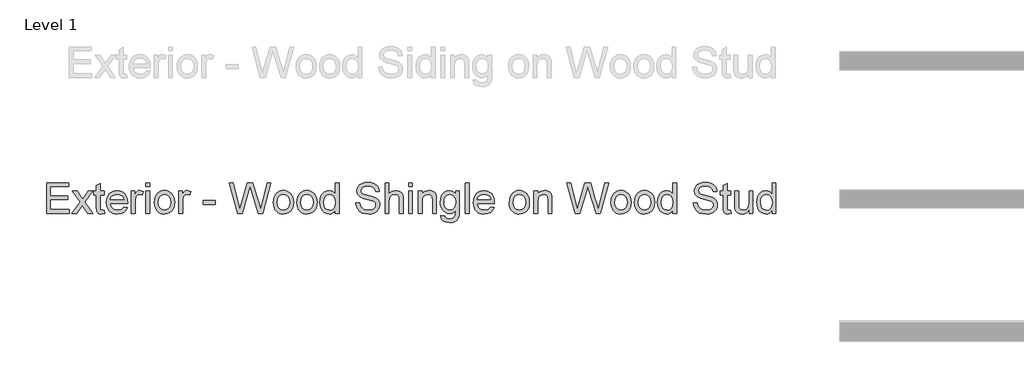
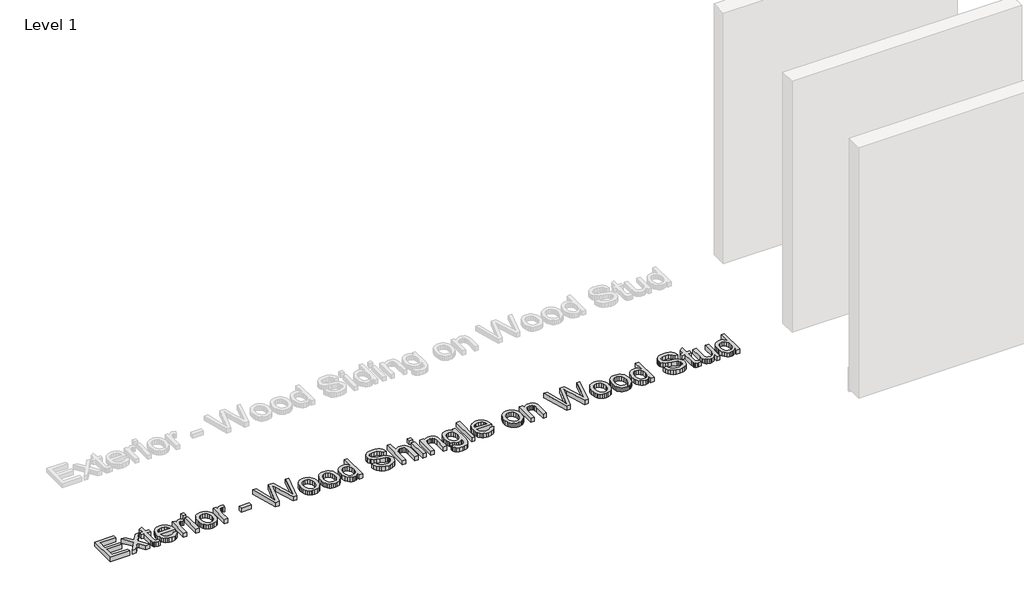
# One storey, part 30 of 42: 1 proxy.
"""IFC4 building model written with IfcOpenShell, lengths in millimetres."""

from ifc_helpers import new_model, si_unit, origin, origin_with_axes, place, context, project, spatial, polyline, outline, extrude, element, save

model = new_model("IFC4")

# Units and contexts
model_context = context("Model", 3, world=origin())
ifc_project = project(units=[si_unit("LENGTHUNIT", "METRE", prefix="MILLI")], contexts=[model_context])

# Site, building, storey
site = spatial("IfcSite", under=ifc_project)
building = spatial("IfcBuilding", under=site)
storey = spatial("IfcBuildingStorey", under=building, Name="Level 1", Elevation=0.0)

# Proxy
placement = place(None, origin())
element("IfcBuildingElementProxy", 1, Name="8\" Arial", ObjectType="8\" Arial", at=placement, inside=storey, context=model_context, shape_type="SweptSolid", body=[
    extrude(outline(polyline([(-7203.1148942, 15956.5861891), (-7203.1148942, 16261.1532832), (-6984.2072954, 16261.1532832), (-6984.2072954, 16223.0823964), (-7165.0440075, 16223.0823964), (-7165.0440075, 16132.6640404), (-6993.7250171, 16132.6640404), (-6993.7250171, 16094.5931536), (-7165.0440075, 16094.5931536), (-7165.0440075, 15994.6570759), (-6979.4484345, 15994.6570759), (-6979.4484345, 15956.5861891), (-7203.1148942, 15956.5861891)])), origin_with_axes(), (0.0, 0.0, 1.0), 50.8),
    extrude(outline(polyline([(-6950.8952695, 15956.5861891), (-6869.5484919, 16069.0142766), (-6946.1364086, 16180.2526488), (-6900.332373, 16180.2526488), (-6863.3768442, 16126.7154643), (-6846.1259737, 16101.4340161), (-6831.1801763, 16122.1053179), (-6789.0940008, 16180.2526488), (-6743.2899651, 16180.2526488), (-6823.7444563, 16069.0142766), (-6746.2642531, 15956.5861891), (-6792.0682888, 15956.5861891), (-6838.6902536, 16024.1768845), (-6847.2413317, 16036.5201799), (-6905.0912338, 15956.5861891), (-6950.8952695, 15956.5861891)])), origin_with_axes(), (0.0, 0.0, 1.0), 50.8),
    extrude(outline(polyline([(-6632.0515929, 15988.3367138), (-6627.292732, 15955.4708311), (-6655.7715399, 15951.8273283), (-6674.044822, 15953.4074188), (-6687.670779, 15958.1476903), (-6697.3000365, 15965.4532853), (-6703.5832199, 15974.7293461), (-6707.0408298, 15990.6603763), (-6708.1933664, 16017.9308797), (-6708.1933664, 16142.1817621), (-6736.7465315, 16142.1817621), (-6736.7465315, 16180.2526488), (-6708.1933664, 16180.2526488), (-6708.1933664, 16234.6077625), (-6670.1224796, 16256.9892799), (-6670.1224796, 16180.2526488), (-6632.0515929, 16180.2526488), (-6632.0515929, 16142.1817621), (-6670.1224796, 16142.1817621), (-6670.1224796, 16019.0462377), (-6668.1148352, 15999.4159367), (-6661.6085801, 15992.4635384), (-6648.6332486, 15989.898215), (-6632.0515929, 15988.3367138)])), origin_with_axes(), (0.0, 0.0, 1.0), 50.8),
    extrude(outline(polyline([(-6437.3844414, 16023.2102409), (-6400.0571267, 16018.4513801), (-6413.5064854, 15990.3257689), (-6434.9678324, 15969.3012704), (-6463.957846, 15956.1958138), (-6499.9932044, 15951.8273283), (-6523.6155576, 15953.7118186), (-6544.6632927, 15959.3652895), (-6563.1364098, 15968.787741), (-6579.0349088, 15981.9791732), (-6591.8197, 15998.5724472), (-6600.9516937, 16018.2004245), (-6606.4308899, 16040.8631051), (-6608.2572886, 16066.5604889), (-6606.4123006, 16093.1292462), (-6600.8773365, 16116.5471171), (-6591.6523963, 16136.8141016), (-6578.73748, 16153.9301998), (-6562.8808069, 16167.5282728), (-6544.8305964, 16177.2411822), (-6524.5868486, 16183.0689278), (-6502.1495632, 16185.0115097), (-6480.434937, 16183.0735751), (-6460.797665, 16177.2597715), (-6443.2377473, 16167.5700988), (-6427.7551839, 16154.004557), (-6415.1167835, 16136.9256374), (-6406.0893546, 16116.6958315), (-6400.6728973, 16093.3151392), (-6398.8674115, 16066.7835605), (-6399.0904831, 16056.5222669), (-6570.1864019, 16056.5222669), (-6563.596495, 16028.0248697), (-6548.2882063, 16007.0747284), (-6526.194823, 15994.1923434), (-6499.2496324, 15989.898215), (-6478.9872952, 15991.8872701), (-6461.9223177, 15997.8544355), (-6448.0546997, 16008.1714971), (-6437.3844414, 16023.2102409)]), holes=[polyline([(-6570.1864019, 16094.5931536), (-6436.9382982, 16094.5931536), (-6442.0875344, 16114.7067764), (-6452.1815244, 16129.0948947), (-6474.3771488, 16142.4791909), (-6502.2982776, 16146.9406229), (-6527.9608065, 16143.3807719), (-6549.1804927, 16132.701219), (-6563.9311024, 16116.0545007), (-6570.1864019, 16094.5931536)])]), origin_with_axes(), (0.0, 0.0, 1.0), 50.8),
    extrude(outline(polyline([(-6360.7965247, 15956.5861891), (-6360.7965247, 16180.2526488), (-6327.4844988, 16180.2526488), (-6327.4844988, 16147.1636945), (-6315.1783821, 16166.3478523), (-6303.838909, 16177.6501468), (-6292.4622573, 16183.1711689), (-6280.0446048, 16185.0115097), (-6261.0835186, 16182.0744002), (-6241.8250036, 16173.263072), (-6254.5400849, 16139.1331168), (-6267.924381, 16144.9887464), (-6281.3086772, 16146.9406229), (-6292.6760342, 16145.0631036), (-6302.8350868, 16139.4305456), (-6311.0422628, 16130.4705029), (-6316.5539903, 16118.6105294), (-6321.182726, 16097.34437), (-6322.725638, 16074.1449234), (-6322.725638, 15956.5861891), (-6360.7965247, 15956.5861891)])), origin_with_axes(), (0.0, 0.0, 1.0), 50.8),
    extrude(outline(polyline([(-6218.0306994, 16223.0823964), (-6218.0306994, 16261.1532832), (-6179.9598126, 16261.1532832), (-6179.9598126, 16223.0823964), (-6218.0306994, 16223.0823964)])), origin_with_axes(), (0.0, 0.0, 1.0), 50.8),
    extrude(outline(polyline([(-6218.0306994, 15956.5861891), (-6218.0306994, 16180.2526488), (-6179.9598126, 16180.2526488), (-6179.9598126, 15956.5861891), (-6218.0306994, 15956.5861891)])), origin_with_axes(), (0.0, 0.0, 1.0), 50.8),
    extrude(outline(polyline([(-6132.3712042, 16068.419419), (-6130.3124392, 16097.386196), (-6124.1361442, 16122.3469788), (-6113.8423192, 16143.3017674), (-6099.4309643, 16160.2505618), (-6084.9220155, 16171.0834765), (-6068.9073334, 16178.8212727), (-6051.386918, 16183.4639504), (-6032.3607692, 16185.0115097), (-6011.3571837, 16183.1270194), (-5992.3658899, 16177.4735484), (-5975.3868878, 16168.0510969), (-5960.4201775, 16154.8596648), (-5948.2046837, 16138.3453952), (-5939.4793309, 16118.9544315), (-5934.2441192, 16096.6867735), (-5932.4990487, 16071.5424214), (-5935.5848725, 16033.0811593), (-5944.842344, 16003.8030116), (-5960.0019183, 15981.876932), (-5980.7940505, 15965.4718746), (-6005.4899358, 15955.2384648), (-6032.3607692, 15951.8273283), (-6053.6710782, 15953.7048476), (-6072.8389704, 15959.3374055), (-6089.8644457, 15968.7250021), (-6104.7475041, 15981.8676373), (-6116.8328729, 15998.5422396), (-6125.4652792, 16018.5257373), (-6130.6447229, 16041.8181304), (-6132.3712042, 16068.419419)]), holes=[polyline([(-6094.3003174, 16068.4937762), (-6089.8946533, 16034.0385083), (-6076.6776608, 16009.4913374), (-6056.7871097, 15994.7964956), (-6032.3607692, 15989.898215), (-6008.0459646, 15994.8243796), (-5988.192592, 16009.6028732), (-5974.9755996, 16034.4753568), (-5970.5699354, 16069.6834914), (-5975.0034835, 16103.134937), (-5988.3041278, 16127.3475005), (-6008.1853843, 16142.0423423), (-6032.3607692, 16146.9406229), (-6056.7871097, 16142.0609316), (-6076.6776608, 16127.4218577), (-6089.8946533, 16102.9304547), (-6094.3003174, 16068.4937762)])]), origin_with_axes(), (0.0, 0.0, 1.0), 50.8),
    extrude(outline(polyline([(-5889.6693011, 15956.5861891), (-5889.6693011, 16180.2526488), (-5856.3572752, 16180.2526488), (-5856.3572752, 16147.1636945), (-5844.0511585, 16166.3478523), (-5832.7116853, 16177.6501468), (-5821.3350336, 16183.1711689), (-5808.9173811, 16185.0115097), (-5789.9562949, 16182.0744002), (-5770.69778, 16173.263072), (-5783.4128613, 16139.1331168), (-5796.7971574, 16144.9887464), (-5810.1814535, 16146.9406229), (-5821.5488106, 16145.0631036), (-5831.7078631, 16139.4305456), (-5839.9150392, 16130.4705029), (-5845.4267667, 16118.6105294), (-5850.0555024, 16097.34437), (-5851.5984143, 16074.1449234), (-5851.5984143, 15956.5861891), (-5889.6693011, 15956.5861891)])), origin_with_axes(), (0.0, 0.0, 1.0), 50.8),
    extrude(outline(polyline([(-5646.967398, 16047.0045452), (-5646.967398, 16085.0754319), (-5527.9958769, 16085.0754319), (-5527.9958769, 16047.0045452), (-5646.967398, 16047.0045452)])), origin_with_axes(), (0.0, 0.0, 1.0), 50.8),
    extrude(outline(polyline([(-5306.9319192, 15956.5861891), (-5389.9889124, 16261.1532832), (-5350.7283104, 16261.1532832), (-5302.5448444, 16060.9836989), (-5287.6734042, 15999.1928651), (-5271.7609633, 16053.8454076), (-5211.3829163, 16261.1532832), (-5154.7970866, 16261.1532832), (-5110.9263381, 16110.8773806), (-5092.1325557, 16055.10948), (-5078.283527, 15999.1928651), (-5063.8582301, 16059.1991261), (-5015.2286208, 16261.1532832), (-4975.9680189, 16261.1532832), (-5059.0993693, 15956.5861891), (-5099.772758, 15956.5861891), (-5172.7915291, 16191.5549433), (-5182.9784656, 16224.3464688), (-5194.4294745, 16184.8627953), (-5260.9791692, 15956.5861891), (-5306.9319192, 15956.5861891)])), origin_with_axes(), (0.0, 0.0, 1.0), 50.8),
    extrude(outline(polyline([(-4952.1737147, 16068.419419), (-4950.1149497, 16097.386196), (-4943.9386547, 16122.3469788), (-4933.6448297, 16143.3017674), (-4919.2334747, 16160.2505618), (-4904.724526, 16171.0834765), (-4888.7098439, 16178.8212727), (-4871.1894284, 16183.4639504), (-4852.1632797, 16185.0115097), (-4831.1596942, 16183.1270194), (-4812.1684004, 16177.4735484), (-4795.1893983, 16168.0510969), (-4780.222688, 16154.8596648), (-4768.0071942, 16138.3453952), (-4759.2818414, 16118.9544315), (-4754.0466297, 16096.6867735), (-4752.3015592, 16071.5424214), (-4755.387383, 16033.0811593), (-4764.6448545, 16003.8030116), (-4779.8044288, 15981.876932), (-4800.596561, 15965.4718746), (-4825.2924463, 15955.2384648), (-4852.1632797, 15951.8273283), (-4873.4735887, 15953.7048476), (-4892.6414808, 15959.3374055), (-4909.6669561, 15968.7250021), (-4924.5500146, 15981.8676373), (-4936.6353834, 15998.5422396), (-4945.2677896, 16018.5257373), (-4950.4472334, 16041.8181304), (-4952.1737147, 16068.419419)]), holes=[polyline([(-4914.1028279, 16068.4937762), (-4909.6971638, 16034.0385083), (-4896.4801713, 16009.4913374), (-4876.5896201, 15994.7964956), (-4852.1632797, 15989.898215), (-4827.8484751, 15994.8243796), (-4807.9951025, 16009.6028732), (-4794.7781101, 16034.4753568), (-4790.3724459, 16069.6834914), (-4794.805994, 16103.134937), (-4808.1066383, 16127.3475005), (-4827.9878948, 16142.0423423), (-4852.1632797, 16146.9406229), (-4876.5896201, 16142.0609316), (-4896.4801713, 16127.4218577), (-4909.6971638, 16102.9304547), (-4914.1028279, 16068.4937762)])]), origin_with_axes(), (0.0, 0.0, 1.0), 50.8),
    extrude(outline(polyline([(-4718.9895333, 16068.419419), (-4716.9307683, 16097.386196), (-4710.7544733, 16122.3469788), (-4700.4606483, 16143.3017674), (-4686.0492933, 16160.2505618), (-4671.5403446, 16171.0834765), (-4655.5256625, 16178.8212727), (-4638.005247, 16183.4639504), (-4618.9790983, 16185.0115097), (-4597.9755128, 16183.1270194), (-4578.984219, 16177.4735484), (-4562.0052169, 16168.0510969), (-4547.0385066, 16154.8596648), (-4534.8230128, 16138.3453952), (-4526.09766, 16118.9544315), (-4520.8624483, 16096.6867735), (-4519.1173778, 16071.5424214), (-4522.2032016, 16033.0811593), (-4531.4606731, 16003.8030116), (-4546.6202474, 15981.876932), (-4567.4123796, 15965.4718746), (-4592.1082649, 15955.2384648), (-4618.9790983, 15951.8273283), (-4640.2894073, 15953.7048476), (-4659.4572994, 15959.3374055), (-4676.4827747, 15968.7250021), (-4691.3658332, 15981.8676373), (-4703.451202, 15998.5422396), (-4712.0836082, 16018.5257373), (-4717.263052, 16041.8181304), (-4718.9895333, 16068.419419)]), holes=[polyline([(-4680.9186465, 16068.4937762), (-4676.5129824, 16034.0385083), (-4663.2959899, 16009.4913374), (-4643.4054387, 15994.7964956), (-4618.9790983, 15989.898215), (-4594.6642937, 15994.8243796), (-4574.8109211, 16009.6028732), (-4561.5939287, 16034.4753568), (-4557.1882645, 16069.6834914), (-4561.6218126, 16103.134937), (-4574.9224569, 16127.3475005), (-4594.8037134, 16142.0423423), (-4618.9790983, 16146.9406229), (-4643.4054387, 16142.0609316), (-4663.2959899, 16127.4218577), (-4676.5129824, 16102.9304547), (-4680.9186465, 16068.4937762)])]), origin_with_axes(), (0.0, 0.0, 1.0), 50.8),
    extrude(outline(polyline([(-4338.2806657, 15956.5861891), (-4338.2806657, 15992.5007171), (-4349.6712594, 15974.7061095), (-4363.4691674, 15961.9956755), (-4379.6743898, 15954.3694151), (-4398.2869266, 15951.8273283), (-4422.8991601, 15955.5080097), (-4445.4293919, 15966.550054), (-4464.5020139, 15984.1820052), (-4478.7414178, 16007.6324074), (-4487.608514, 16035.9532062), (-4490.5642127, 16068.1963474), (-4487.8408802, 16100.0398186), (-4479.6708828, 16128.7974659), (-4466.0635151, 16152.8334311), (-4447.0280717, 16170.5118555), (-4424.0052234, 16181.3865961), (-4398.435641, 16185.0115097), (-4379.8091623, 16182.4183023), (-4363.3390423, 16174.6386802), (-4349.3784779, 16162.7136441), (-4338.2806657, 16147.6841949), (-4338.2806657, 16261.1532832), (-4300.2097789, 16261.1532832), (-4300.2097789, 15956.5861891), (-4338.2806657, 15956.5861891)]), holes=[polyline([(-4452.4933259, 16068.3450618), (-4448.1991976, 16033.9083832), (-4435.3168126, 16009.4169802), (-4416.5973873, 15994.7779063), (-4394.7921382, 15989.898215), (-4372.9961837, 15994.5548347), (-4354.7507856, 16008.5246938), (-4342.3981957, 16032.0680425), (-4338.2806657, 16065.4451309), (-4342.4725529, 16101.9359272), (-4355.0482144, 16127.2359647), (-4373.7583451, 16142.0144584), (-4396.3536394, 16146.9406229), (-4418.3819601, 16142.209646), (-4436.4321706, 16128.0167153), (-4448.4780371, 16103.6368481), (-4452.4933259, 16068.3450618)])]), origin_with_axes(), (0.0, 0.0, 1.0), 50.8),
    extrude(outline(polyline([(-4133.6496493, 16061.2811277), (-4095.5787626, 16061.2811277), (-4091.210277, 16040.154388), (-4083.3098245, 16023.1730623), (-4070.9851185, 16009.6958197), (-4053.3438726, 15999.0813293), (-4031.7802844, 15992.1939936), (-4007.6885514, 15989.898215), (-3986.4781599, 15991.6363146), (-3967.907449, 15996.8506133), (-3952.8594105, 16005.1042626), (-3942.2170361, 16015.9604139), (-3935.8873794, 16028.4245396), (-3933.7774939, 16041.5021123), (-3935.3575844, 16054.2450776), (-3940.0978559, 16065.2592379), (-3949.7271134, 16074.6561292), (-3965.9741618, 16082.5472871), (-4021.4074549, 16097.0841198), (-4057.79601, 16106.7040827), (-4081.0791084, 16115.859313), (-4100.0309, 16128.6673408), (-4113.4616694, 16144.1894065), (-4121.4643631, 16162.0909025), (-4124.1319277, 16182.0372216), (-4120.8323269, 16204.3350872), (-4110.9335245, 16225.1272194), (-4094.6957708, 16242.749876), (-4072.379316, 16255.5393145), (-4045.5921344, 16263.3189367), (-4015.9422006, 16265.912144), (-3983.8198899, 16263.1981062), (-3955.7128681, 16255.0559927), (-3932.6249572, 16241.6531073), (-3915.5599797, 16223.1567536), (-3904.7595963, 16200.7194683), (-3900.4654679, 16175.493788), (-3938.5363547, 16175.493788), (-3945.5259316, 16198.2099128), (-3960.0999429, 16214.6056755), (-3982.8718356, 16224.5323618), (-4014.4550566, 16227.8412573), (-4046.7818496, 16224.5695404), (-4068.9588847, 16214.7543899), (-4081.7855019, 16200.3105037), (-4086.0610409, 16183.1525796), (-4083.030985, 16168.5228004), (-4073.9408172, 16156.7557734), (-4052.4515862, 16146.2342295), (-4011.7781974, 16135.489614), (-3969.8035576, 16125.2840882), (-3944.4105736, 16116.3798134), (-3922.7075656, 16102.5679634), (-3907.5665806, 16085.5215751), (-3898.6716005, 16065.4265416), (-3895.7066071, 16042.4687559), (-3899.1177437, 16018.9997644), (-3909.3511534, 15996.9249705), (-3925.9885771, 15977.9267057), (-3948.6117554, 15963.6873018), (-3975.8171962, 15954.7923216), (-4006.2014073, 15951.8273283), (-4043.5008381, 15955.0246879), (-4074.2010674, 15964.6167668), (-4098.6552918, 15980.6407435), (-4117.216708, 16003.1337968), (-4129.1324494, 16030.5344252), (-4133.6496493, 16061.2811277)])), origin_with_axes(), (0.0, 0.0, 1.0), 50.8),
    extrude(outline(polyline([(-3843.3591378, 15956.5861891), (-3843.3591378, 16261.1532832), (-3805.288251, 16261.1532832), (-3805.288251, 16149.1713389), (-3791.30445, 16164.8514136), (-3775.6011387, 16176.051467), (-3758.1783171, 16182.771499), (-3739.0359852, 16185.0115097), (-3716.0410209, 16182.5670167), (-3696.2805948, 16175.2335378), (-3680.7213506, 16163.5873412), (-3670.3299318, 16148.2046953), (-3664.4743022, 16127.068661), (-3662.5224257, 16098.1622992), (-3662.5224257, 15956.5861891), (-3700.5933125, 15956.5861891), (-3700.5933125, 16094.2213676), (-3703.6233684, 16118.0528504), (-3712.7135362, 16134.374256), (-3727.3619047, 16143.7990312), (-3747.0665629, 16146.9406229), (-3763.1556022, 16144.8214427), (-3778.2594086, 16138.463902), (-3790.7700076, 16128.4814478), (-3799.0794248, 16115.487527), (-3803.7360445, 16098.2180671), (-3805.288251, 16075.4089958), (-3805.288251, 15956.5861891), (-3843.3591378, 15956.5861891)])), origin_with_axes(), (0.0, 0.0, 1.0), 50.8),
    extrude(outline(polyline([(-3610.1749564, 16223.0823964), (-3610.1749564, 16261.1532832), (-3572.1040697, 16261.1532832), (-3572.1040697, 16223.0823964), (-3610.1749564, 16223.0823964)])), origin_with_axes(), (0.0, 0.0, 1.0), 50.8),
    extrude(outline(polyline([(-3610.1749564, 15956.5861891), (-3610.1749564, 16180.2526488), (-3572.1040697, 16180.2526488), (-3572.1040697, 15956.5861891), (-3610.1749564, 15956.5861891)])), origin_with_axes(), (0.0, 0.0, 1.0), 50.8),
    extrude(outline(polyline([(-3514.9977395, 15956.5861891), (-3514.9977395, 16180.2526488), (-3476.9268528, 16180.2526488), (-3476.9268528, 16149.0226245), (-3463.7005657, 16164.7677618), (-3447.8160087, 16176.0142884), (-3429.2731818, 16182.7622043), (-3408.0720849, 16185.0115097), (-3389.3061864, 16183.1990529), (-3372.1203784, 16177.7616826), (-3357.7880279, 16169.3779082), (-3347.5825021, 16158.7262392), (-3336.1686718, 16130.7307532), (-3334.1610274, 16093.9239388), (-3334.1610274, 15956.5861891), (-3372.2319142, 15956.5861891), (-3372.2319142, 16088.793292), (-3376.618989, 16122.4771039), (-3382.6883955, 16132.5060313), (-3392.1224654, 16140.2856534), (-3404.2148051, 16145.2768805), (-3418.2590214, 16146.9406229), (-3440.556887, 16143.2041736), (-3459.5644464, 16131.9948256), (-3467.1604992, 16122.8442426), (-3472.5862512, 16110.3382909), (-3476.9268528, 16075.2602814), (-3476.9268528, 15956.5861891), (-3514.9977395, 15956.5861891)])), origin_with_axes(), (0.0, 0.0, 1.0), 50.8),
    extrude(outline(polyline([(-3291.3312798, 15937.5507457), (-3253.2603931, 15932.7918849), (-3249.0592112, 15920.8947328), (-3240.9170977, 15912.7154407), (-3224.9117103, 15906.3579), (-3203.961569, 15904.2387198), (-3181.6172302, 15906.6367395), (-3164.9983958, 15913.8307987), (-3153.4730297, 15925.3561648), (-3146.4090956, 15940.7481054), (-3143.8065936, 15985.1393542), (-3156.4752017, 15972.6473445), (-3170.6123645, 15963.7244804), (-3186.218082, 15958.3707619), (-3203.2923542, 15956.5861891), (-3224.1658146, 15958.6635434), (-3242.5436615, 15964.8956063), (-3258.4258948, 15975.2823778), (-3271.8125146, 15989.8238578), (-3282.433976, 16007.269916), (-3290.0207341, 16026.370422), (-3294.572789, 16047.1253756), (-3296.0901407, 16069.534777), (-3293.3668082, 16100.2721848), (-3285.1968108, 16128.5372157), (-3271.8682825, 16152.489529), (-3253.6693577, 16170.2887839), (-3231.2227777, 16181.3308282), (-3205.1512842, 16185.0115097), (-3187.347382, 16182.929508), (-3171.1886328, 16176.6835032), (-3156.6750367, 16166.2734951), (-3143.8065936, 16151.6994837), (-3143.8065936, 16180.2526488), (-3105.7357069, 16180.2526488), (-3105.7357069, 15987.1469986), (-3108.3382089, 15942.5605621), (-3116.145715, 15913.1987625), (-3129.5950736, 15893.7264706), (-3149.1231335, 15878.8085572), (-3174.3023406, 15869.3280141), (-3204.705141, 15866.1678331), (-3240.1270525, 15870.6199705), (-3268.0202974, 15883.9763826), (-3278.5255757, 15894.0029864), (-3285.9124988, 15906.2742482), (-3290.1810669, 15920.790168), (-3291.3312798, 15937.5507457)]), holes=[polyline([(-3258.0192539, 16072.137279), (-3253.9574918, 16037.2172786), (-3241.7722055, 16013.2091974), (-3223.4524502, 15999.2951063), (-3200.987281, 15994.6570759), (-3178.6894154, 15999.2672223), (-3160.2767136, 16013.0976616), (-3147.9241236, 16036.7990194), (-3143.8065936, 16071.021921), (-3148.0449541, 16104.0272235), (-3160.7600354, 16127.7936437), (-3179.4422821, 16142.1538781), (-3201.5821386, 16146.9406229), (-3223.3223251, 16142.2282353), (-3241.5491339, 16128.0910725), (-3253.9017239, 16104.677849), (-3258.0192539, 16072.137279)])]), origin_with_axes(), (0.0, 0.0, 1.0), 50.8),
    extrude(outline(polyline([(-3048.6293767, 15956.5861891), (-3048.6293767, 16261.1532832), (-3010.55849, 16261.1532832), (-3010.55849, 15956.5861891), (-3048.6293767, 15956.5861891)])), origin_with_axes(), (0.0, 0.0, 1.0), 50.8),
    extrude(outline(polyline([(-2796.8558952, 16023.2102409), (-2759.5285804, 16018.4513801), (-2772.9779391, 15990.3257689), (-2794.4392861, 15969.3012704), (-2823.4292998, 15956.1958138), (-2859.4646581, 15951.8273283), (-2883.0870113, 15953.7118186), (-2904.1347465, 15959.3652895), (-2922.6078635, 15968.787741), (-2938.5063625, 15981.9791732), (-2951.2911537, 15998.5724472), (-2960.4231474, 16018.2004245), (-2965.9023436, 16040.8631051), (-2967.7287424, 16066.5604889), (-2965.8837543, 16093.1292462), (-2960.3487902, 16116.5471171), (-2951.12385, 16136.8141016), (-2938.2089337, 16153.9301998), (-2922.3522606, 16167.5282728), (-2904.3020502, 16177.2411822), (-2884.0583023, 16183.0689278), (-2861.621017, 16185.0115097), (-2839.9063907, 16183.0735751), (-2820.2691187, 16177.2597715), (-2802.709201, 16167.5700988), (-2787.2266377, 16154.004557), (-2774.5882372, 16136.9256374), (-2765.5608083, 16116.6958315), (-2760.144351, 16093.3151392), (-2758.3388652, 16066.7835605), (-2758.5619368, 16056.5222669), (-2929.6578556, 16056.5222669), (-2923.0679487, 16028.0248697), (-2907.75966, 16007.0747284), (-2885.6662767, 15994.1923434), (-2858.7210861, 15989.898215), (-2838.4587489, 15991.8872701), (-2821.3937714, 15997.8544355), (-2807.5261535, 16008.1714971), (-2796.8558952, 16023.2102409)]), holes=[polyline([(-2929.6578556, 16094.5931536), (-2796.4097519, 16094.5931536), (-2801.5589881, 16114.7067764), (-2811.6529781, 16129.0948947), (-2833.8486025, 16142.4791909), (-2861.7697314, 16146.9406229), (-2887.4322603, 16143.3807719), (-2908.6519464, 16132.701219), (-2923.4025561, 16116.0545007), (-2929.6578556, 16094.5931536)])]), origin_with_axes(), (0.0, 0.0, 1.0), 50.8),
    extrude(outline(polyline([(-2610.814179, 16068.419419), (-2608.755414, 16097.386196), (-2602.579119, 16122.3469788), (-2592.2852941, 16143.3017674), (-2577.8739391, 16160.2505618), (-2563.3649903, 16171.0834765), (-2547.3503082, 16178.8212727), (-2529.8298928, 16183.4639504), (-2510.8037441, 16185.0115097), (-2489.8001585, 16183.1270194), (-2470.8088647, 16177.4735484), (-2453.8298627, 16168.0510969), (-2438.8631524, 16154.8596648), (-2426.6476585, 16138.3453952), (-2417.9223057, 16118.9544315), (-2412.6870941, 16096.6867735), (-2410.9420235, 16071.5424214), (-2414.0278473, 16033.0811593), (-2423.2853188, 16003.8030116), (-2438.4448931, 15981.876932), (-2459.2370254, 15965.4718746), (-2483.9329107, 15955.2384648), (-2510.8037441, 15951.8273283), (-2532.114053, 15953.7048476), (-2551.2819452, 15959.3374055), (-2568.3074205, 15968.7250021), (-2583.1904789, 15981.8676373), (-2595.2758477, 15998.5422396), (-2603.908254, 16018.5257373), (-2609.0876977, 16041.8181304), (-2610.814179, 16068.419419)]), holes=[polyline([(-2572.7432922, 16068.4937762), (-2568.3376281, 16034.0385083), (-2555.1206357, 16009.4913374), (-2535.2300845, 15994.7964956), (-2510.8037441, 15989.898215), (-2486.4889394, 15994.8243796), (-2466.6355668, 16009.6028732), (-2453.4185744, 16034.4753568), (-2449.0129103, 16069.6834914), (-2453.4464584, 16103.134937), (-2466.7471026, 16127.3475005), (-2486.6283592, 16142.0423423), (-2510.8037441, 16146.9406229), (-2535.2300845, 16142.0609316), (-2555.1206357, 16127.4218577), (-2568.3376281, 16102.9304547), (-2572.7432922, 16068.4937762)])]), origin_with_axes(), (0.0, 0.0, 1.0), 50.8),
    extrude(outline(polyline([(-2368.1122759, 15956.5861891), (-2368.1122759, 16180.2526488), (-2330.0413892, 16180.2526488), (-2330.0413892, 16149.0226245), (-2316.8151021, 16164.7677618), (-2300.9305451, 16176.0142884), (-2282.3877182, 16182.7622043), (-2261.1866213, 16185.0115097), (-2242.4207228, 16183.1990529), (-2225.2349148, 16177.7616826), (-2210.9025643, 16169.3779082), (-2200.6970385, 16158.7262392), (-2189.2832082, 16130.7307532), (-2187.2755638, 16093.9239388), (-2187.2755638, 15956.5861891), (-2225.3464506, 15956.5861891), (-2225.3464506, 16088.793292), (-2229.7335254, 16122.4771039), (-2235.8029319, 16132.5060313), (-2245.2370018, 16140.2856534), (-2257.3293415, 16145.2768805), (-2271.3735578, 16146.9406229), (-2293.6714234, 16143.2041736), (-2312.6789828, 16131.9948256), (-2320.2750356, 16122.8442426), (-2325.7007876, 16110.3382909), (-2330.0413892, 16075.2602814), (-2330.0413892, 15956.5861891), (-2368.1122759, 15956.5861891)])), origin_with_axes(), (0.0, 0.0, 1.0), 50.8),
    extrude(outline(polyline([(-1956.6938844, 15956.5861891), (-2039.7508776, 16261.1532832), (-2000.4902757, 16261.1532832), (-1952.3068096, 16060.9836989), (-1937.4353695, 15999.1928651), (-1921.5229285, 16053.8454076), (-1861.1448815, 16261.1532832), (-1804.5590518, 16261.1532832), (-1760.6883034, 16110.8773806), (-1741.8945209, 16055.10948), (-1728.0454923, 15999.1928651), (-1713.6201954, 16059.1991261), (-1664.9905861, 16261.1532832), (-1625.7299841, 16261.1532832), (-1708.8613345, 15956.5861891), (-1749.5347233, 15956.5861891), (-1822.5534944, 16191.5549433), (-1832.7404309, 16224.3464688), (-1844.1914398, 16184.8627953), (-1910.7411344, 15956.5861891), (-1956.6938844, 15956.5861891)])), origin_with_axes(), (0.0, 0.0, 1.0), 50.8),
    extrude(outline(polyline([(-1601.9356799, 16068.419419), (-1599.8769149, 16097.386196), (-1593.7006199, 16122.3469788), (-1583.4067949, 16143.3017674), (-1568.99544, 16160.2505618), (-1554.4864912, 16171.0834765), (-1538.4718091, 16178.8212727), (-1520.9513937, 16183.4639504), (-1501.925245, 16185.0115097), (-1480.9216594, 16183.1270194), (-1461.9303656, 16177.4735484), (-1444.9513636, 16168.0510969), (-1429.9846533, 16154.8596648), (-1417.7691594, 16138.3453952), (-1409.0438066, 16118.9544315), (-1403.808595, 16096.6867735), (-1402.0635244, 16071.5424214), (-1405.1493482, 16033.0811593), (-1414.4068197, 16003.8030116), (-1429.566394, 15981.876932), (-1450.3585263, 15965.4718746), (-1475.0544116, 15955.2384648), (-1501.925245, 15951.8273283), (-1523.2355539, 15953.7048476), (-1542.4034461, 15959.3374055), (-1559.4289214, 15968.7250021), (-1574.3119798, 15981.8676373), (-1586.3973486, 15998.5422396), (-1595.0297549, 16018.5257373), (-1600.2091986, 16041.8181304), (-1601.9356799, 16068.419419)]), holes=[polyline([(-1563.8647931, 16068.4937762), (-1559.459129, 16034.0385083), (-1546.2421366, 16009.4913374), (-1526.3515854, 15994.7964956), (-1501.925245, 15989.898215), (-1477.6104403, 15994.8243796), (-1457.7570677, 16009.6028732), (-1444.5400753, 16034.4753568), (-1440.1344112, 16069.6834914), (-1444.5679593, 16103.134937), (-1457.8686035, 16127.3475005), (-1477.7498601, 16142.0423423), (-1501.925245, 16146.9406229), (-1526.3515854, 16142.0609316), (-1546.2421366, 16127.4218577), (-1559.459129, 16102.9304547), (-1563.8647931, 16068.4937762)])]), origin_with_axes(), (0.0, 0.0, 1.0), 50.8),
    extrude(outline(polyline([(-1368.7514985, 16068.419419), (-1366.6927335, 16097.386196), (-1360.5164385, 16122.3469788), (-1350.2226136, 16143.3017674), (-1335.8112586, 16160.2505618), (-1321.3023098, 16171.0834765), (-1305.2876277, 16178.8212727), (-1287.7672123, 16183.4639504), (-1268.7410636, 16185.0115097), (-1247.737478, 16183.1270194), (-1228.7461842, 16177.4735484), (-1211.7671822, 16168.0510969), (-1196.8004719, 16154.8596648), (-1184.584978, 16138.3453952), (-1175.8596252, 16118.9544315), (-1170.6244136, 16096.6867735), (-1168.879343, 16071.5424214), (-1171.9651668, 16033.0811593), (-1181.2226383, 16003.8030116), (-1196.3822126, 15981.876932), (-1217.1743449, 15965.4718746), (-1241.8702302, 15955.2384648), (-1268.7410636, 15951.8273283), (-1290.0513725, 15953.7048476), (-1309.2192647, 15959.3374055), (-1326.24474, 15968.7250021), (-1341.1277984, 15981.8676373), (-1353.2131672, 15998.5422396), (-1361.8455735, 16018.5257373), (-1367.0250172, 16041.8181304), (-1368.7514985, 16068.419419)]), holes=[polyline([(-1330.6806117, 16068.4937762), (-1326.2749476, 16034.0385083), (-1313.0579552, 16009.4913374), (-1293.167404, 15994.7964956), (-1268.7410636, 15989.898215), (-1244.4262589, 15994.8243796), (-1224.5728863, 16009.6028732), (-1211.3558939, 16034.4753568), (-1206.9502298, 16069.6834914), (-1211.3837779, 16103.134937), (-1224.6844221, 16127.3475005), (-1244.5656787, 16142.0423423), (-1268.7410636, 16146.9406229), (-1293.167404, 16142.0609316), (-1313.0579552, 16127.4218577), (-1326.2749476, 16102.9304547), (-1330.6806117, 16068.4937762)])]), origin_with_axes(), (0.0, 0.0, 1.0), 50.8),
    extrude(outline(polyline([(-988.0426309, 15956.5861891), (-988.0426309, 15992.5007171), (-999.4332246, 15974.7061095), (-1013.2311327, 15961.9956755), (-1029.4363551, 15954.3694151), (-1048.0488919, 15951.8273283), (-1072.6611253, 15955.5080097), (-1095.1913571, 15966.550054), (-1114.2639791, 15984.1820052), (-1128.503383, 16007.6324074), (-1137.3704792, 16035.9532062), (-1140.326178, 16068.1963474), (-1137.6028455, 16100.0398186), (-1129.432848, 16128.7974659), (-1115.8254803, 16152.8334311), (-1096.7900369, 16170.5118555), (-1073.7671887, 16181.3865961), (-1048.1976063, 16185.0115097), (-1029.5711275, 16182.4183023), (-1013.1010076, 16174.6386802), (-999.1404431, 16162.7136441), (-988.0426309, 16147.6841949), (-988.0426309, 16261.1532832), (-949.9717442, 16261.1532832), (-949.9717442, 15956.5861891), (-988.0426309, 15956.5861891)]), holes=[polyline([(-1102.2552912, 16068.3450618), (-1097.9611629, 16033.9083832), (-1085.0787778, 16009.4169802), (-1066.3593526, 15994.7779063), (-1044.5541035, 15989.898215), (-1022.758149, 15994.5548347), (-1004.5127509, 16008.5246938), (-992.1601609, 16032.0680425), (-988.0426309, 16065.4451309), (-992.2345181, 16101.9359272), (-1004.8101797, 16127.2359647), (-1023.5203103, 16142.0144584), (-1046.1156047, 16146.9406229), (-1068.1439254, 16142.209646), (-1086.1941358, 16128.0167153), (-1098.2400024, 16103.6368481), (-1102.2552912, 16068.3450618)])]), origin_with_axes(), (0.0, 0.0, 1.0), 50.8),
    extrude(outline(polyline([(-783.4116146, 16061.2811277), (-745.3407278, 16061.2811277), (-740.9722423, 16040.154388), (-733.0717897, 16023.1730623), (-720.7470837, 16009.6958197), (-703.1058378, 15999.0813293), (-681.5422496, 15992.1939936), (-657.4505166, 15989.898215), (-636.2401251, 15991.6363146), (-617.6694142, 15996.8506133), (-602.6213757, 16005.1042626), (-591.9790014, 16015.9604139), (-585.6493447, 16028.4245396), (-583.5394591, 16041.5021123), (-585.1195496, 16054.2450776), (-589.8598212, 16065.2592379), (-599.4890787, 16074.6561292), (-615.736127, 16082.5472871), (-671.1694201, 16097.0841198), (-707.5579752, 16106.7040827), (-730.8410737, 16115.859313), (-749.7928652, 16128.6673408), (-763.2236346, 16144.1894065), (-771.2263283, 16162.0909025), (-773.8938929, 16182.0372216), (-770.5942921, 16204.3350872), (-760.6954898, 16225.1272194), (-744.4577361, 16242.749876), (-722.1412812, 16255.5393145), (-695.3540997, 16263.3189367), (-665.7041659, 16265.912144), (-633.5818552, 16263.1981062), (-605.4748333, 16255.0559927), (-582.3869225, 16241.6531073), (-565.3219449, 16223.1567536), (-554.5215615, 16200.7194683), (-550.2274332, 16175.493788), (-588.29832, 16175.493788), (-595.2878968, 16198.2099128), (-609.8619082, 16214.6056755), (-632.6338009, 16224.5323618), (-664.2170219, 16227.8412573), (-696.5438149, 16224.5695404), (-718.72085, 16214.7543899), (-731.5474671, 16200.3105037), (-735.8230061, 16183.1525796), (-732.7929502, 16168.5228004), (-723.7027824, 16156.7557734), (-702.2135514, 16146.2342295), (-661.5401626, 16135.489614), (-619.5655228, 16125.2840882), (-594.1725388, 16116.3798134), (-572.4695309, 16102.5679634), (-557.3285459, 16085.5215751), (-548.4335657, 16065.4265416), (-545.4685723, 16042.4687559), (-548.8797089, 16018.9997644), (-559.1131187, 15996.9249705), (-575.7505423, 15977.9267057), (-598.3737206, 15963.6873018), (-625.5791615, 15954.7923216), (-655.9633726, 15951.8273283), (-693.2628034, 15955.0246879), (-723.9630326, 15964.6167668), (-748.417257, 15980.6407435), (-766.9786732, 16003.1337968), (-778.8944146, 16030.5344252), (-783.4116146, 16061.2811277)])), origin_with_axes(), (0.0, 0.0, 1.0), 50.8),
    extrude(outline(polyline([(-412.2204687, 15988.3367138), (-407.4616079, 15955.4708311), (-435.9404157, 15951.8273283), (-454.2136978, 15953.4074188), (-467.8396548, 15958.1476903), (-477.4689123, 15965.4532853), (-483.7520958, 15974.7293461), (-487.2097056, 15990.6603763), (-488.3622422, 16017.9308797), (-488.3622422, 16142.1817621), (-516.9154073, 16142.1817621), (-516.9154073, 16180.2526488), (-488.3622422, 16180.2526488), (-488.3622422, 16234.6077625), (-450.2913555, 16256.9892799), (-450.2913555, 16180.2526488), (-412.2204687, 16180.2526488), (-412.2204687, 16142.1817621), (-450.2913555, 16142.1817621), (-450.2913555, 16019.0462377), (-448.283711, 15999.4159367), (-441.777456, 15992.4635384), (-428.8021245, 15989.898215), (-412.2204687, 15988.3367138)])), origin_with_axes(), (0.0, 0.0, 1.0), 50.8),
    extrude(outline(polyline([(-231.3837566, 15956.5861891), (-231.3837566, 15995.0288619), (-245.158428, 15976.1281909), (-261.2009941, 15962.6277117), (-279.5114547, 15954.5274241), (-300.08981, 15951.8273283), (-318.632637, 15953.7234369), (-335.8928022, 15959.4117627), (-350.373867, 15967.9628408), (-360.5793928, 15978.4472061), (-367.4481392, 15991.1808767), (-371.9188659, 16006.4798708), (-374.1495819, 16041.8738983), (-374.1495819, 16180.2526488), (-336.0786952, 16180.2526488), (-336.0786952, 16059.7939837), (-333.773622, 16020.9795249), (-328.2247159, 16008.0320773), (-318.7162888, 15998.1890429), (-305.880377, 15991.970922), (-290.3490167, 15989.898215), (-273.92537, 15992.0173952), (-258.5613134, 15998.3749359), (-245.8927054, 16008.385274), (-237.5554043, 16021.4628467), (-232.9266685, 16039.3736374), (-231.3837566, 16063.8836297), (-231.3837566, 16180.2526488), (-193.3128698, 16180.2526488), (-193.3128698, 15956.5861891), (-231.3837566, 15956.5861891)])), origin_with_axes(), (0.0, 0.0, 1.0), 50.8),
    extrude(outline(polyline([(-2.958436, 15956.5861891), (-2.958436, 15992.5007171), (-14.3490297, 15974.7061095), (-28.1469378, 15961.9956755), (-44.3521602, 15954.3694151), (-62.964697, 15951.8273283), (-87.5769304, 15955.5080097), (-110.1071622, 15966.550054), (-129.1797842, 15984.1820052), (-143.4191882, 16007.6324074), (-152.2862843, 16035.9532062), (-155.2419831, 16068.1963474), (-152.5186506, 16100.0398186), (-144.3486532, 16128.7974659), (-130.7412854, 16152.8334311), (-111.7058421, 16170.5118555), (-88.6829938, 16181.3865961), (-63.1134114, 16185.0115097), (-44.4869326, 16182.4183023), (-28.0168127, 16174.6386802), (-14.0562482, 16162.7136441), (-2.958436, 16147.6841949), (-2.958436, 16261.1532832), (35.1124507, 16261.1532832), (35.1124507, 15956.5861891), (-2.958436, 15956.5861891)]), holes=[polyline([(-117.1710963, 16068.3450618), (-112.876968, 16033.9083832), (-99.994583, 16009.4169802), (-81.2751577, 15994.7779063), (-59.4699086, 15989.898215), (-37.6739541, 15994.5548347), (-19.428556, 16008.5246938), (-7.075966, 16032.0680425), (-2.958436, 16065.4451309), (-7.1503232, 16101.9359272), (-19.7259848, 16127.2359647), (-38.4361154, 16142.0144584), (-61.0314098, 16146.9406229), (-83.0597305, 16142.209646), (-101.109941, 16128.0167153), (-113.1558075, 16103.6368481), (-117.1710963, 16068.3450618)])]), origin_with_axes(), (0.0, 0.0, 1.0), 50.8),
])

save(model, "model.ifc")

# Revit data of these elements
# Element 1 (IfcBuildingElementProxy, "8\" Arial")
#   Phase Created = New Construction
